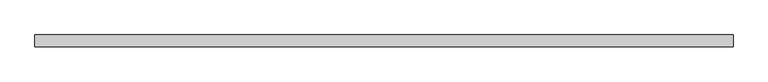
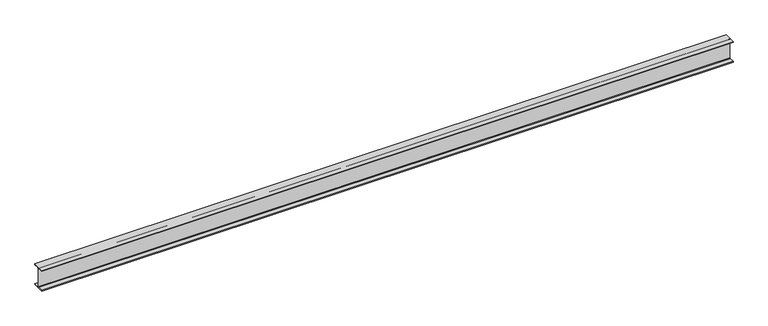
"""IFC4 building model written with IfcOpenShell, lengths in millimetres: beam geometry, Old_Steel Beam_H-KSD3502 : H_SB_ASB_H-350×175x7x11."""

from ifc_helpers import new_model, si_unit, point, frame, frame_2d, origin, place, context, project, spatial, polyline, circle_curve, trimmed, segment, composite_curve, outline, extrude, source, transform, mapped, element, save


def beam_34d84ffc(model_context):
    return source(origin(), model_context, "Body", "SweptSolid", [
        extrude(outline(composite_curve([segment(polyline([(82.5, -141.5), (82.5, -151.7), (-82.5, -151.7), (-82.5, -141.5), (-11.9, -141.5)]), True, "CONTINUOUS"), segment(trimmed(circle_curve(frame_2d((-11.9, -132.6)), 8.9), [point((-11.9, -141.5))], [point((-3.0, -132.6))], True, "CARTESIAN"), True, "CONTINUOUS"), segment(polyline([(-3.0, -132.6), (-3.0, 132.6)]), True, "CONTINUOUS"), segment(trimmed(circle_curve(frame_2d((-11.9, 132.6)), 8.9), [point((-3.0, 132.6))], [point((-11.9, 141.5))], True, "CARTESIAN"), True, "CONTINUOUS"), segment(polyline([(-11.9, 141.5), (-82.5, 141.5), (-82.5, 151.7), (82.5, 151.7), (82.5, 141.5), (11.9, 141.5)]), True, "CONTINUOUS"), segment(trimmed(circle_curve(frame_2d((11.9, 132.6)), 8.9), [point((11.9, 141.5))], [point((3.0, 132.6))], True, "CARTESIAN"), True, "CONTINUOUS"), segment(polyline([(3.0, 132.6), (3.0, -132.6)]), True, "CONTINUOUS"), segment(trimmed(circle_curve(frame_2d((11.9, -132.6)), 8.9), [point((3.0, -132.6))], [point((11.9, -141.5))], True, "CARTESIAN"), True, "CONTINUOUS"), segment(polyline([(11.9, -141.5), (82.5, -141.5)]), True, "CONTINUOUS")], self_intersect=False)), frame((-4837.3, 0.0, 0.0), z_axis=(1.0, 0.0, 0.0), x_axis=(0.0, 1.0, 0.0)), (0.0, 0.0, 1.0), 9699.6),
    ])


if __name__ == "__main__":
    model = new_model("IFC4")
    model_context = context("Model", 3, world=origin())
    ifc_project = project(units=[si_unit("LENGTHUNIT", "METRE", prefix="MILLI")], contexts=[model_context])
    site = spatial("IfcSite", under=ifc_project)
    building = spatial("IfcBuilding", under=site)
    placement = place(None, origin())
    beam_shape = beam_34d84ffc(model_context)
    element("IfcBeam", 1, ObjectType="Old_Steel Beam_H-KSD3502 : H_SB_ASB_H-350×175x7x11", at=placement, inside=building, context=model_context, shape_type="MappedRepresentation", body=[
        mapped(beam_shape, transform((0.0, 0.0, 0.0), x_axis=(1.0, 0.0, 0.0), y_axis=(0.0, 1.0, 0.0), z_axis=(0.0, 0.0, 1.0))),
    ])
    save(model, "model.ifc")

# Revit data of these elements
# Type "Old_Steel Beam_H-KSD3502 : H_SB_ASB_H-350×175x7x11"
#   Width = 17.5 cm
#   Web Thickness = 0.7 cm
#   Web Fillet = 1.4 cm
#   Warping Constant = 282290.0 cm⁶
#   Torsional Moment of Inertia = 19.4042 cm⁴
#   Torsional Modulus = 1.0 cm³
#   Section Area = 63.14 cm²
#   Plastic Modulus weak axis = 174.0 cm³
#   Plastic Modulus strong axis = 868.0 cm³
#   Perimeter = 1.36 m²/m
#   Nominal Weight = 49.60 kgf/m
#   Moment of Inertia weak axis = 984.00 cm⁴
#   Moment of Inertia strong axis = 13600.00 cm⁴
#   Height = 35.0 cm
#   Flange Thickness = 1.1 cm
#   Elastic Modulus weak axis = 112.0 cm³
#   Elastic Modulus strong axis = 775.0 cm³
#   Centroid Vertical = 17.5 cm
#   Centroid Horizontal = 8.75 cm
#   Length [instance default] = 1.5240 m
#   Structural Material [instance default] = Steel, 45-345
#   Assembly Code = ""
# Element 1 (IfcBeam, "Old_Steel Beam_H-KSD3502 : H_SB_ASB_H-350×175x7x11")
#   Structural Material = none
# Materials
#   "Steel, 45-345": class "Metal", colour RGB 189 187 185, transparency 0, Description = "Steel 345 MPa", Cost = 0
